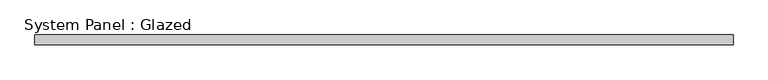
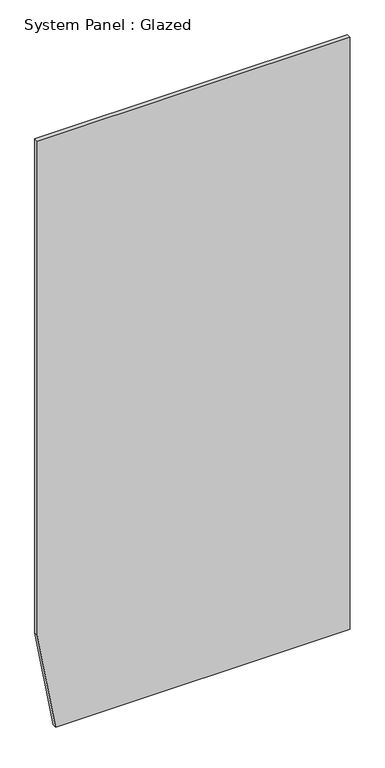
"""IFC4 building model written with IfcOpenShell, lengths in millimetres: plate geometry, System Panel : Glazed."""

import ifcopenshell
import ifcopenshell.guid

model = None  # the IFC model being written
_history = None  # IfcOwnerHistory: only IFC2X3 demands one
_inside = {}  # id of a spatial element -> (the spatial element, [elements in it])
_under = {}  # id of a project, library or spatial element -> (it, [spatial elements below it])
_declared = {}  # id of a project -> (the project, [libraries it declares])
_typed = {}  # id of a type object -> (the type object, [elements of that type])
_made_of = {}  # id of a material, layer set ... -> (it, [elements and type objects made of it])


def new_model(schema):
    """Start an empty IFC model of exactly this schema.

    Asked for "IFC4X3", IfcOpenShell would pick the latest addendum, in which some entities
    have other attributes; the version numbers below select the first issue.
    IFC2X3 requires an IfcOwnerHistory on every rooted entity: one is made here for all.
    """
    global model, _history
    if schema == "IFC4X3":
        model = ifcopenshell.file(schema_version=(4, 3, 0, 0))
    else:
        model = ifcopenshell.file(schema=schema)
    _inside.clear()
    _under.clear()
    _declared.clear()
    _typed.clear()
    _made_of.clear()
    _history = None
    if model.schema == "IFC2X3":
        org = make("IfcOrganization", Name="unknown")
        user = make(
            "IfcPersonAndOrganization",
            ThePerson=make("IfcPerson", FamilyName="unknown"),
            TheOrganization=org,
        )
        app = make(
            "IfcApplication",
            ApplicationDeveloper=org,
            Version="unknown",
            ApplicationFullName="unknown",
            ApplicationIdentifier="unknown",
        )
        _history = make(
            "IfcOwnerHistory",
            OwningUser=user,
            OwningApplication=app,
            ChangeAction="ADDED",
            CreationDate=0,
        )
    return model


def make(cls, **values):
    """One entity of the class cls with the attributes given. An attribute that is None is left unset."""
    return model.create_entity(
        cls, **{name: value for name, value in values.items() if value is not None}
    )


def rooted(cls, **values):
    """An entity with a GlobalId (a new one), such as an element, a storey or a relation."""
    return make(cls, GlobalId=ifcopenshell.guid.new(), OwnerHistory=_history, **values)


def si_unit(unit_type, name, prefix=None):
    """IfcSIUnit, for example si_unit("LENGTHUNIT", "METRE", prefix="MILLI")."""
    return make("IfcSIUnit", UnitType=unit_type, Prefix=prefix, Name=name)


def assignment(units):
    """IfcUnitAssignment: the units of a project."""
    return None if units is None else make("IfcUnitAssignment", Units=units)


def point(xyz):
    """IfcCartesianPoint."""
    return None if xyz is None else make("IfcCartesianPoint", Coordinates=xyz)


def direction(xyz):
    """IfcDirection."""
    return None if xyz is None else make("IfcDirection", DirectionRatios=xyz)


def frame(location, z_axis=None, x_axis=None):
    """IfcAxis2Placement3D, a coordinate frame: its origin and axes. An axis left out is left unset."""
    return make(
        "IfcAxis2Placement3D",
        Location=point(location),
        Axis=direction(z_axis),
        RefDirection=direction(x_axis),
    )


def origin():
    """The frame at (0, 0, 0) with its axes left unset."""
    return frame((0.0, 0.0, 0.0))


def place(relative_to, where):
    """IfcLocalPlacement: puts the frame where relative to a parent placement (None: the world)."""
    return make(
        "IfcLocalPlacement", PlacementRelTo=relative_to, RelativePlacement=where
    )


def context(
    kind, dimensions, precision=None, world=None, true_north=None, identifier=None
):
    """IfcGeometricRepresentationContext, for example the 3D "Model" context."""
    return make(
        "IfcGeometricRepresentationContext",
        ContextIdentifier=identifier,
        ContextType=kind,
        CoordinateSpaceDimension=dimensions,
        Precision=precision,
        WorldCoordinateSystem=world,
        TrueNorth=true_north,
    )


def project(units=None, contexts=None):
    """IfcProject with its units and contexts."""
    return rooted(
        "IfcProject",
        Name="project",
        RepresentationContexts=contexts,
        UnitsInContext=assignment(units),
    )


def spatial(cls, under=None, at=None, **own):
    """A site, building, storey or space (cls), placed at a placement, below another one or the project."""
    s = rooted(cls, ObjectPlacement=at, **own)
    if under is not None:
        _under.setdefault(under.id(), (under, []))[1].append(s)
    return s


def polyline(points):
    """IfcPolyline through the points."""
    return make("IfcPolyline", Points=[point(p) for p in points])


def outline(outer, holes=None, kind="AREA"):
    """IfcArbitraryClosedProfileDef: a profile drawn as a closed curve; with holes, ...WithVoids."""
    if holes is None:
        return make("IfcArbitraryClosedProfileDef", ProfileType=kind, OuterCurve=outer)
    return make(
        "IfcArbitraryProfileDefWithVoids",
        ProfileType=kind,
        OuterCurve=outer,
        InnerCurves=holes,
    )


def extrude(swept, where, along, depth):
    """IfcExtrudedAreaSolid: the profile swept, set in the frame where, extruded along a direction by depth."""
    return make(
        "IfcExtrudedAreaSolid",
        SweptArea=swept,
        Position=where,
        ExtrudedDirection=direction(along),
        Depth=depth,
    )


def shape(context_of_items, identifier, shape_type, items):
    """IfcShapeRepresentation: the items that make up one representation, for example the "Body"."""
    return make(
        "IfcShapeRepresentation",
        ContextOfItems=context_of_items,
        RepresentationIdentifier=identifier,
        RepresentationType=shape_type,
        Items=items,
    )


def source(mapping_origin, context_of_items, identifier, shape_type, items):
    """IfcRepresentationMap: a shape defined once, which mapped items show again and again."""
    return make(
        "IfcRepresentationMap",
        MappingOrigin=mapping_origin,
        MappedRepresentation=shape(context_of_items, identifier, shape_type, items),
    )


def transform(
    local_origin,
    x_axis=None,
    y_axis=None,
    z_axis=None,
    scale=None,
    scale2=None,
    scale3=None,
    uniform=True,
):
    """IfcCartesianTransformationOperator3D, or its non-uniform kind. x_axis, y_axis, z_axis: its Axis1, 2, 3."""
    if uniform:
        return make(
            "IfcCartesianTransformationOperator3D",
            Axis1=direction(x_axis),
            Axis2=direction(y_axis),
            LocalOrigin=point(local_origin),
            Scale=scale,
            Axis3=direction(z_axis),
        )
    return make(
        "IfcCartesianTransformationOperator3DnonUniform",
        Axis1=direction(x_axis),
        Axis2=direction(y_axis),
        LocalOrigin=point(local_origin),
        Scale=scale,
        Axis3=direction(z_axis),
        Scale2=scale2,
        Scale3=scale3,
    )


def mapped(mapping_source, mapping_target):
    """IfcMappedItem: shows the shape of a source again, moved by a transform."""
    return make(
        "IfcMappedItem", MappingSource=mapping_source, MappingTarget=mapping_target
    )


def made_of(thing, what):
    """Note that an element or type object is made of a material, layer set ...; save() writes the relation."""
    if what is not None:
        _made_of.setdefault(what.id(), (what, []))[1].append(thing)
    return thing


def element(
    cls,
    number,
    at=None,
    inside=None,
    cuts=None,
    type_object=None,
    material=None,
    context=None,
    identifier="Body",
    shape_type=None,
    held_by="IfcProductDefinitionShape",
    body=None,
    shapes=None,
    **own,
):
    """One element of the class cls, such as IfcWall. Its Tag is "e" and its number.

    at: its placement. inside: the storey or other place that contains it. cuts: it is an
    opening in that element (IfcRelVoidsElement). A single representation is given by context,
    identifier, shape_type and body (its items); several are given by shapes. held_by: the class
    of the entity that holds the representations. save() writes the other relations.
    """
    e = rooted(cls, Tag="e%d" % number, ObjectPlacement=at, **own)
    if body is not None:
        shapes = [shape(context, identifier, shape_type, body)]
    if shapes is not None:
        e.Representation = make(held_by, Representations=shapes)
    if inside is not None:
        _inside.setdefault(inside.id(), (inside, []))[1].append(e)
    if cuts is not None:
        rooted(
            "IfcRelVoidsElement", RelatingBuildingElement=cuts, RelatedOpeningElement=e
        )
    if type_object is not None:
        _typed.setdefault(type_object.id(), (type_object, []))[1].append(e)
    return made_of(e, material)


def aggregate(whole, parts):
    """IfcRelAggregates: a whole, such as a stair, and the parts it consists of."""
    return rooted("IfcRelAggregates", RelatingObject=whole, RelatedObjects=parts)


def save(model, path):
    """Write the relations noted so far, then the file.

    IfcRelAggregates (storeys below a building ...), IfcRelContainedInSpatialStructure (elements
    in a storey), IfcRelDefinesByType, IfcRelAssociatesMaterial and IfcRelDeclares: one each for
    every whole, place, type object, material and project.
    """
    for whole, parts in _under.values():
        aggregate(whole, parts)
    for where, things in _inside.values():
        rooted(
            "IfcRelContainedInSpatialStructure",
            RelatedElements=things,
            RelatingStructure=where,
        )
    for kind, things in _typed.values():
        rooted("IfcRelDefinesByType", RelatedObjects=things, RelatingType=kind)
    for what, things in _made_of.values():
        rooted("IfcRelAssociatesMaterial", RelatedObjects=things, RelatingMaterial=what)
    for by, libraries in _declared.values():
        rooted("IfcRelDeclares", RelatingContext=by, RelatedDefinitions=libraries)
    model.write(path)


def system_panel_glazed_866ab655(model_context):
    return source(origin(), model_context, "Body", "SweptSolid", [
        extrude(outline(polyline([(0.0, -808.3993064), (0.0, 914.4), (3657.6, 914.4), (3657.6, -914.4), (603.4561394, -914.4), (0.0, -808.3993064)])), frame((0.0, -44.45, 0.0), z_axis=(0.0, 1.0, 0.0), x_axis=(0.0, 0.0, 1.0)), (0.0, 0.0, 1.0), 25.4),
    ])


if __name__ == "__main__":
    model = new_model("IFC4")
    model_context = context("Model", 3, world=origin())
    ifc_project = project(units=[si_unit("LENGTHUNIT", "METRE", prefix="MILLI")], contexts=[model_context])
    site = spatial("IfcSite", under=ifc_project)
    building = spatial("IfcBuilding", under=site)
    placement = place(None, origin())
    system_panel_glazed_shape = system_panel_glazed_866ab655(model_context)
    element("IfcPlate", 1, ObjectType="System Panel : Glazed", at=placement, inside=building, context=model_context, shape_type="MappedRepresentation", body=[
        mapped(system_panel_glazed_shape, transform((0.0, 0.0, 0.0), x_axis=(1.0, 0.0, 0.0), y_axis=(0.0, 1.0, 0.0), z_axis=(0.0, 0.0, 1.0))),
    ])
    save(model, "model.ifc")

# Revit data of these elements
# Type "System Panel : Glazed"
#   Construction Type Id = "GSP4R"
#   Analytic Construction = "1/8 in Pilkington single glazing"
#   Visual Light Transmittance = 0.9
#   Solar Heat Gain Coefficient = 0.86
#   Heat Transfer Coefficient (U) = 1.18115 BTU/(h·ft²·°F)
#   Define Thermal Properties by = 1
# Element 1 (IfcPlate, "System Panel : Glazed")
#   Materials on its faces: "Glass"
# Materials
#   "Glass": class "Glass", colour RGB 0 128 192, transparency 0.75, Description = "Soda Lime Glass", Cost = 0
